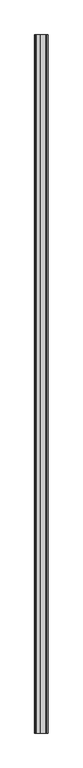
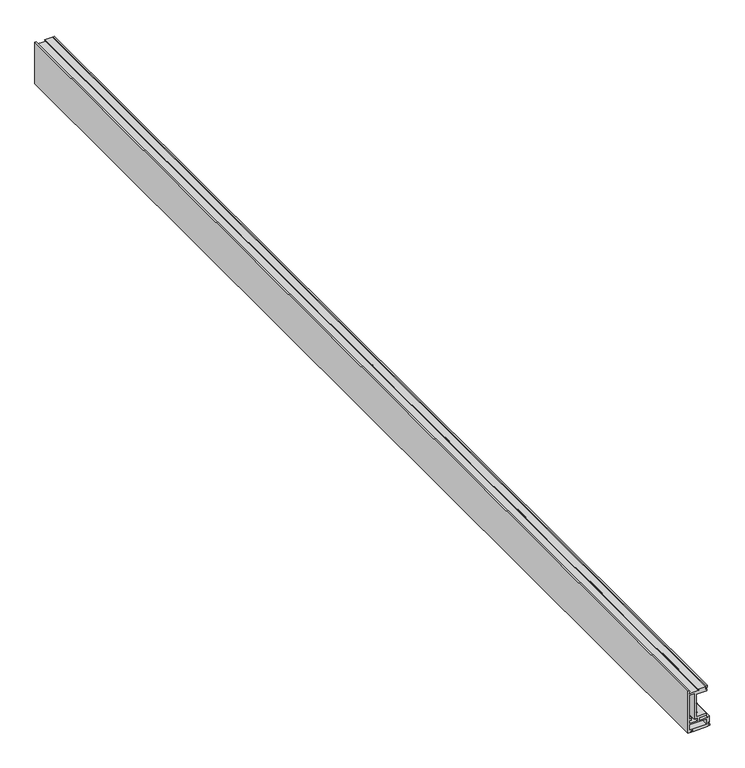
"""IFC4 building model written with IfcOpenShell, lengths in millimetres: proxy geometry, Door frame13:Door frame012:296427 : Door frame13:Door frame012:296427."""

from ifc_helpers import new_model, si_unit, frame, origin, place, context, project, spatial, polyline, outline, extrude, source, transform, mapped, element, save


def generic_models_5b0aadc3(model_context):
    return source(origin(), model_context, "Body", "SweptSolid", [
        extrude(outline(polyline([(36610.4200435, 20316.5176028), (36608.9977225, 20316.5176028), (36608.9977225, 20301.526561), (36613.8237225, 20301.526561), (36613.8237225, 20314.3475213), (36616.9987225, 20314.3475213), (36616.9987225, 20296.5167248), (36623.9157731, 20296.5167248), (36624.8727225, 20297.9197967), (36625.8290531, 20296.5167248), (36640.6803935, 20296.5167248), (36641.6367241, 20297.9197967), (36642.5936735, 20296.5167248), (36658.8030324, 20296.5167248), (36658.8030324, 20315.2567898), (36662.4618113, 20315.2567898), (36661.0188583, 20312.7575219), (36666.3421883, 20312.7575219), (36665.4695635, 20316.0142021), (36668.703989, 20316.2975799), (36667.561659, 20313.9577207), (36667.7957063, 20312.7575219), (36667.7957063, 20299.1443768), (36666.5824658, 20299.1443768), (36666.5824658, 20300.6611682), (36664.6229889, 20300.6611682), (36664.6229889, 20283.8674379), (36666.7220494, 20283.8674379), (36668.7089205, 20285.0145584), (36669.4492947, 20284.5948669), (36669.4492947, 20281.8355213), (36591.6236909, 20281.8355213), (36591.6236909, 20287.4176882), (36592.8950628, 20287.4176882), (36592.8950628, 20286.5345213), (36594.1652793, 20286.5345213), (36594.1652793, 20291.1065208), (36592.8950628, 20291.1065208), (36592.8950628, 20290.2233539), (36591.6240434, 20290.2233539), (36591.6240434, 20317.1919802), (36593.5561506, 20317.1919802), (36593.5561506, 20318.3743151), (36592.4137824, 20320.7141744), (36595.6482078, 20320.4307966), (36594.775583, 20317.1741164), (36600.1211436, 20317.1741164), (36598.5843732, 20319.6926029), (36610.4200435, 20319.6926029), (36610.4200435, 20316.5176028)]), holes=[polyline([(36608.9977225, 20298.3502522), (36608.9977225, 20285.0152522), (36613.8237225, 20285.0152522), (36613.8237225, 20288.1855213), (36616.9987225, 20288.1855213), (36616.9987225, 20285.0105213), (36661.4479889, 20285.0105213), (36661.4479889, 20293.3417248), (36613.8237225, 20293.3417248), (36613.8237225, 20298.3502522), (36608.9977225, 20298.3502522)]), polyline([(36605.8183749, 20285.0105213), (36605.8183749, 20314.6523266), (36596.3988909, 20314.6523266), (36596.3988909, 20285.0105213), (36605.8183749, 20285.0105213)])]), frame((0.0, -774.5581156, 0.0), z_axis=(0.0, 1.0, 0.0), x_axis=(0.0, 0.0, 1.0)), (0.0, 0.0, 1.0), 1999.85),
    ])


if __name__ == "__main__":
    model = new_model("IFC4")
    model_context = context("Model", 3, world=origin())
    ifc_project = project(units=[si_unit("LENGTHUNIT", "METRE", prefix="MILLI")], contexts=[model_context])
    site = spatial("IfcSite", under=ifc_project)
    building = spatial("IfcBuilding", under=site)
    placement = place(None, origin())
    generic_models_shape = generic_models_5b0aadc3(model_context)
    element("IfcBuildingElementProxy", 1, Name="Door frame13:Door frame012:296427 : Door frame13:Door frame012:296427", ObjectType="Door frame13:Door frame012:296427 : Door frame13:Door frame012:296427", at=placement, inside=building, context=model_context, shape_type="MappedRepresentation", body=[
        mapped(generic_models_shape, transform((0.0, 0.0, 0.0), x_axis=(1.0, 0.0, 0.0), y_axis=(0.0, 1.0, 0.0), z_axis=(0.0, 0.0, 1.0))),
    ])
    save(model, "model.ifc")

# Revit data of these elements
# Type "Door frame13:Door frame012:296427 : Door frame13:Door frame012:296427"
#   NameOverride = "Door frame13:Door frame012:296427"
#   ObjectTypeOverride = "Door frame13:Door frame012"
#   Reference = "Door frame012"
#   Category = "Generic Models"
#   Tag = "296427"
# Element 1 (IfcBuildingElementProxy, "Door frame13:Door frame012:296427 : Door frame13:Door frame012:296427")
#   Materials on its faces: "FLEETWOOD SERIES T-3200 SINGLE SWING DOOR FRAME"
# Materials
#   "FLEETWOOD SERIES T-3200 SINGLE SWING DOOR FRAME": class "Unassigned", colour RGB 128 128 128, transparency 0, Cost = 0
